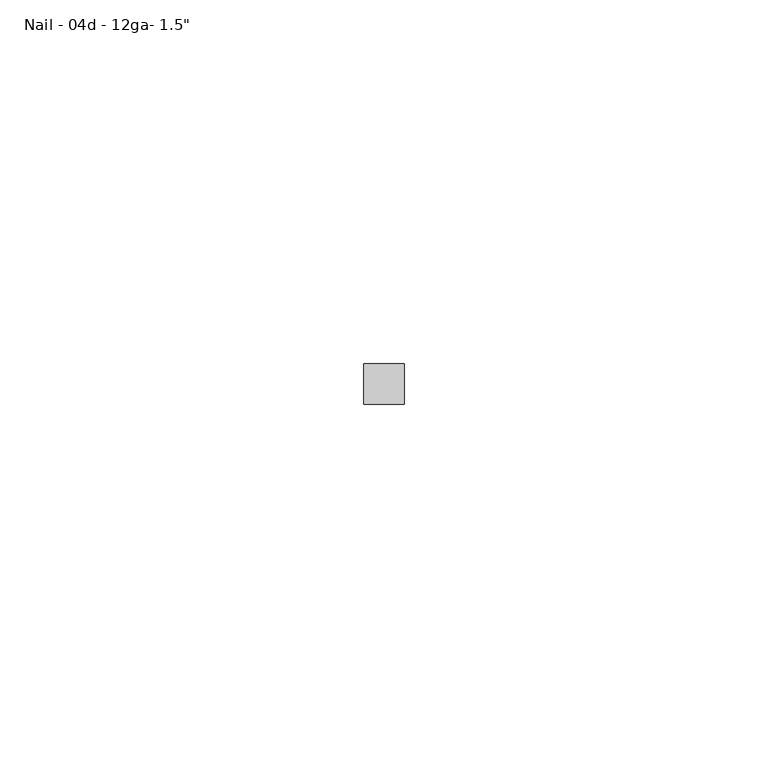
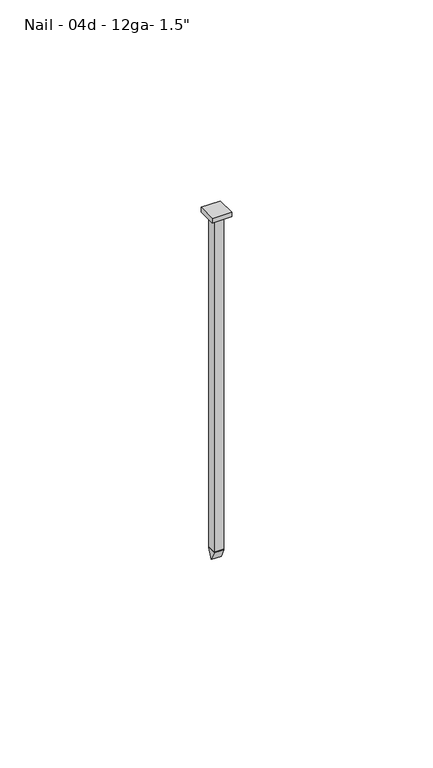
"""IFC4 building model written with IfcOpenShell, lengths in millimetres: fastener geometry."""

import ifcopenshell
import ifcopenshell.guid

model = None  # the IFC model being written
_history = None  # IfcOwnerHistory: only IFC2X3 demands one
_inside = {}  # id of a spatial element -> (the spatial element, [elements in it])
_under = {}  # id of a project, library or spatial element -> (it, [spatial elements below it])
_declared = {}  # id of a project -> (the project, [libraries it declares])
_typed = {}  # id of a type object -> (the type object, [elements of that type])
_made_of = {}  # id of a material, layer set ... -> (it, [elements and type objects made of it])


def new_model(schema):
    """Start an empty IFC model of exactly this schema.

    Asked for "IFC4X3", IfcOpenShell would pick the latest addendum, in which some entities
    have other attributes; the version numbers below select the first issue.
    IFC2X3 requires an IfcOwnerHistory on every rooted entity: one is made here for all.
    """
    global model, _history
    if schema == "IFC4X3":
        model = ifcopenshell.file(schema_version=(4, 3, 0, 0))
    else:
        model = ifcopenshell.file(schema=schema)
    _inside.clear()
    _under.clear()
    _declared.clear()
    _typed.clear()
    _made_of.clear()
    _history = None
    if model.schema == "IFC2X3":
        org = make("IfcOrganization", Name="unknown")
        user = make(
            "IfcPersonAndOrganization",
            ThePerson=make("IfcPerson", FamilyName="unknown"),
            TheOrganization=org,
        )
        app = make(
            "IfcApplication",
            ApplicationDeveloper=org,
            Version="unknown",
            ApplicationFullName="unknown",
            ApplicationIdentifier="unknown",
        )
        _history = make(
            "IfcOwnerHistory",
            OwningUser=user,
            OwningApplication=app,
            ChangeAction="ADDED",
            CreationDate=0,
        )
    return model


def make(cls, **values):
    """One entity of the class cls with the attributes given. An attribute that is None is left unset."""
    return model.create_entity(
        cls, **{name: value for name, value in values.items() if value is not None}
    )


def rooted(cls, **values):
    """An entity with a GlobalId (a new one), such as an element, a storey or a relation."""
    return make(cls, GlobalId=ifcopenshell.guid.new(), OwnerHistory=_history, **values)


def si_unit(unit_type, name, prefix=None):
    """IfcSIUnit, for example si_unit("LENGTHUNIT", "METRE", prefix="MILLI")."""
    return make("IfcSIUnit", UnitType=unit_type, Prefix=prefix, Name=name)


def assignment(units):
    """IfcUnitAssignment: the units of a project."""
    return None if units is None else make("IfcUnitAssignment", Units=units)


def point(xyz):
    """IfcCartesianPoint."""
    return None if xyz is None else make("IfcCartesianPoint", Coordinates=xyz)


def direction(xyz):
    """IfcDirection."""
    return None if xyz is None else make("IfcDirection", DirectionRatios=xyz)


def frame(location, z_axis=None, x_axis=None):
    """IfcAxis2Placement3D, a coordinate frame: its origin and axes. An axis left out is left unset."""
    return make(
        "IfcAxis2Placement3D",
        Location=point(location),
        Axis=direction(z_axis),
        RefDirection=direction(x_axis),
    )


def origin():
    """The frame at (0, 0, 0) with its axes left unset."""
    return frame((0.0, 0.0, 0.0))


def origin_with_axes():
    """The frame at (0, 0, 0) with the z axis (0, 0, 1) and the x axis (1, 0, 0) written out."""
    return frame((0.0, 0.0, 0.0), z_axis=(0.0, 0.0, 1.0), x_axis=(1.0, 0.0, 0.0))


def place(relative_to, where):
    """IfcLocalPlacement: puts the frame where relative to a parent placement (None: the world)."""
    return make(
        "IfcLocalPlacement", PlacementRelTo=relative_to, RelativePlacement=where
    )


def context(
    kind, dimensions, precision=None, world=None, true_north=None, identifier=None
):
    """IfcGeometricRepresentationContext, for example the 3D "Model" context."""
    return make(
        "IfcGeometricRepresentationContext",
        ContextIdentifier=identifier,
        ContextType=kind,
        CoordinateSpaceDimension=dimensions,
        Precision=precision,
        WorldCoordinateSystem=world,
        TrueNorth=true_north,
    )


def project(units=None, contexts=None):
    """IfcProject with its units and contexts."""
    return rooted(
        "IfcProject",
        Name="project",
        RepresentationContexts=contexts,
        UnitsInContext=assignment(units),
    )


def spatial(cls, under=None, at=None, **own):
    """A site, building, storey or space (cls), placed at a placement, below another one or the project."""
    s = rooted(cls, ObjectPlacement=at, **own)
    if under is not None:
        _under.setdefault(under.id(), (under, []))[1].append(s)
    return s


def polyline(points):
    """IfcPolyline through the points."""
    return make("IfcPolyline", Points=[point(p) for p in points])


def outline(outer, holes=None, kind="AREA"):
    """IfcArbitraryClosedProfileDef: a profile drawn as a closed curve; with holes, ...WithVoids."""
    if holes is None:
        return make("IfcArbitraryClosedProfileDef", ProfileType=kind, OuterCurve=outer)
    return make(
        "IfcArbitraryProfileDefWithVoids",
        ProfileType=kind,
        OuterCurve=outer,
        InnerCurves=holes,
    )


def extrude(swept, where, along, depth):
    """IfcExtrudedAreaSolid: the profile swept, set in the frame where, extruded along a direction by depth."""
    return make(
        "IfcExtrudedAreaSolid",
        SweptArea=swept,
        Position=where,
        ExtrudedDirection=direction(along),
        Depth=depth,
    )


def shape(context_of_items, identifier, shape_type, items):
    """IfcShapeRepresentation: the items that make up one representation, for example the "Body"."""
    return make(
        "IfcShapeRepresentation",
        ContextOfItems=context_of_items,
        RepresentationIdentifier=identifier,
        RepresentationType=shape_type,
        Items=items,
    )


def source(mapping_origin, context_of_items, identifier, shape_type, items):
    """IfcRepresentationMap: a shape defined once, which mapped items show again and again."""
    return make(
        "IfcRepresentationMap",
        MappingOrigin=mapping_origin,
        MappedRepresentation=shape(context_of_items, identifier, shape_type, items),
    )


def transform(
    local_origin,
    x_axis=None,
    y_axis=None,
    z_axis=None,
    scale=None,
    scale2=None,
    scale3=None,
    uniform=True,
):
    """IfcCartesianTransformationOperator3D, or its non-uniform kind. x_axis, y_axis, z_axis: its Axis1, 2, 3."""
    if uniform:
        return make(
            "IfcCartesianTransformationOperator3D",
            Axis1=direction(x_axis),
            Axis2=direction(y_axis),
            LocalOrigin=point(local_origin),
            Scale=scale,
            Axis3=direction(z_axis),
        )
    return make(
        "IfcCartesianTransformationOperator3DnonUniform",
        Axis1=direction(x_axis),
        Axis2=direction(y_axis),
        LocalOrigin=point(local_origin),
        Scale=scale,
        Axis3=direction(z_axis),
        Scale2=scale2,
        Scale3=scale3,
    )


def mapped(mapping_source, mapping_target):
    """IfcMappedItem: shows the shape of a source again, moved by a transform."""
    return make(
        "IfcMappedItem", MappingSource=mapping_source, MappingTarget=mapping_target
    )


def made_of(thing, what):
    """Note that an element or type object is made of a material, layer set ...; save() writes the relation."""
    if what is not None:
        _made_of.setdefault(what.id(), (what, []))[1].append(thing)
    return thing


def element(
    cls,
    number,
    at=None,
    inside=None,
    cuts=None,
    type_object=None,
    material=None,
    context=None,
    identifier="Body",
    shape_type=None,
    held_by="IfcProductDefinitionShape",
    body=None,
    shapes=None,
    **own,
):
    """One element of the class cls, such as IfcWall. Its Tag is "e" and its number.

    at: its placement. inside: the storey or other place that contains it. cuts: it is an
    opening in that element (IfcRelVoidsElement). A single representation is given by context,
    identifier, shape_type and body (its items); several are given by shapes. held_by: the class
    of the entity that holds the representations. save() writes the other relations.
    """
    e = rooted(cls, Tag="e%d" % number, ObjectPlacement=at, **own)
    if body is not None:
        shapes = [shape(context, identifier, shape_type, body)]
    if shapes is not None:
        e.Representation = make(held_by, Representations=shapes)
    if inside is not None:
        _inside.setdefault(inside.id(), (inside, []))[1].append(e)
    if cuts is not None:
        rooted(
            "IfcRelVoidsElement", RelatingBuildingElement=cuts, RelatedOpeningElement=e
        )
    if type_object is not None:
        _typed.setdefault(type_object.id(), (type_object, []))[1].append(e)
    return made_of(e, material)


def aggregate(whole, parts):
    """IfcRelAggregates: a whole, such as a stair, and the parts it consists of."""
    return rooted("IfcRelAggregates", RelatingObject=whole, RelatedObjects=parts)


def save(model, path):
    """Write the relations noted so far, then the file.

    IfcRelAggregates (storeys below a building ...), IfcRelContainedInSpatialStructure (elements
    in a storey), IfcRelDefinesByType, IfcRelAssociatesMaterial and IfcRelDeclares: one each for
    every whole, place, type object, material and project.
    """
    for whole, parts in _under.values():
        aggregate(whole, parts)
    for where, things in _inside.values():
        rooted(
            "IfcRelContainedInSpatialStructure",
            RelatedElements=things,
            RelatingStructure=where,
        )
    for kind, things in _typed.values():
        rooted("IfcRelDefinesByType", RelatedObjects=things, RelatingType=kind)
    for what, things in _made_of.values():
        rooted("IfcRelAssociatesMaterial", RelatedObjects=things, RelatingMaterial=what)
    for by, libraries in _declared.values():
        rooted("IfcRelDeclares", RelatingContext=by, RelatedDefinitions=libraries)
    model.write(path)


def fastener_92d45581(model_context):
    return source(origin(), model_context, "Body", "SweptSolid", [
        extrude(outline(polyline([(0.0, -104.3686), (-1.3843, -101.6), (1.3843, -101.6), (0.0, -104.3686)])), frame((-1.3843, 0.0, 0.0), z_axis=(1.0, 0.0, 0.0), x_axis=(0.0, 1.0, 0.0)), (0.0, 0.0, 1.0), 2.7686),
        extrude(outline(polyline([(-2.7686, -2.7686), (-2.7686, 2.7686), (2.7686, 2.7686), (2.7686, -2.7686), (-2.7686, -2.7686)])), origin_with_axes(), (0.0, 0.0, 1.0), 1.3843),
        extrude(outline(polyline([(-1.3843, 1.3843), (1.3843, 1.3843), (1.3843, -1.3843), (-1.3843, -1.3843), (-1.3843, 1.3843)])), frame((0.0, 0.0, -101.6), z_axis=(0.0, 0.0, 1.0), x_axis=(1.0, 0.0, 0.0)), (0.0, 0.0, 1.0), 101.6),
    ])


if __name__ == "__main__":
    model = new_model("IFC4")
    model_context = context("Model", 3, world=origin())
    ifc_project = project(units=[si_unit("LENGTHUNIT", "METRE", prefix="MILLI")], contexts=[model_context])
    site = spatial("IfcSite", under=ifc_project)
    building = spatial("IfcBuilding", under=site)
    placement = place(None, origin())
    fastener_shape = fastener_92d45581(model_context)
    element("IfcFastener", 1, ObjectType="060523 - W_P_C - Fastenings - Generic - SQUARE : Nail - 04d - 12ga- 1.5\"", at=placement, inside=building, context=model_context, shape_type="MappedRepresentation", body=[
        mapped(fastener_shape, transform((0.0, 0.0, 0.0), x_axis=(1.0, 0.0, 0.0), y_axis=(0.0, 1.0, 0.0), z_axis=(0.0, 0.0, 1.0))),
    ])
    save(model, "model.ifc")

# Revit data of these elements
# Type "060523 - W_P_C - Fastenings - Generic - SQUARE : Nail - 04d - 12ga- 1.5\""
#   Washer_Thickness = 0' - 0.00333"
#   Washer Radius = 0' - 0.0645"
#   Washer Offset - Head = 0' - 0"
#   Washer Offset = 0' - 0"
#   Thickness_of_Substrate [instance default] = 0' - 1"
#   Side = 0' - 0 37/64"
#   Radius = 0' - 0.0545"
#   Length [instance default] = 0' - 1 1/2"
#   Head Size = 0' - 1"
#   Head Radius = 0' - 0 1/2"
#   Head Height = 0' - 0.01"
#   Double Diameter = 0' - 0.218"
#   Diameter = 0' - 0.109"
#   Default Elevation = 4' - 0"
#   Washer_Nut_Visibility = no
#   Washer_Head_Visibility = no
#   Round_Head_Visibility = yes
#   Point Visibility = yes
#   Nut_Visibility = no
#   Hex_Head_Visiblilty = no
#   Washer Material = none
#   Bolt Material (Size) = AT SILL - FASTENER AT 24" O.C.
# Element 1 (IfcFastener, "060523 - W_P_C - Fastenings - Generic - SQUARE : Nail - 04d - 12ga- 1.5\"")
#   Length = 0' - 4"
# Materials
#   "AT SILL - FASTENER AT 24\" O.C.": class "Generic", colour RGB 120 120 120, transparency 0, Cost = 0
